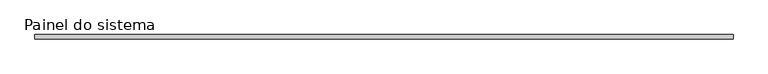
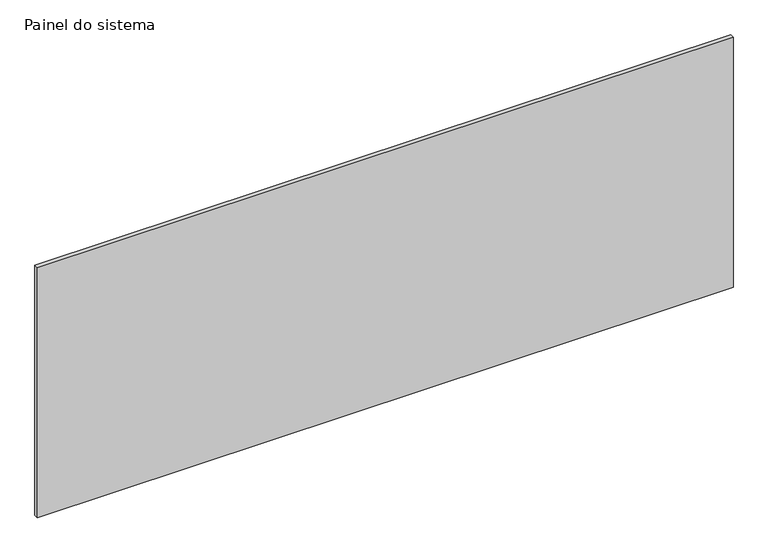
"""IFC4 building model written with IfcOpenShell, lengths in millimetres: plate geometry, Painel do sistema : Envidraçado."""

from ifc_helpers import new_model, si_unit, origin, origin_with_axes, place, context, project, spatial, polyline, outline, extrude, source, transform, mapped, element, save


def painel_do_sistema_4da26680(model_context):
    return source(origin(), model_context, "Body", "SweptSolid", [
        extrude(outline(polyline([(1975.0000075, 24.5), (-1975.0000075, 24.5), (-1975.0000075, 49.5), (1975.0000075, 49.5), (1975.0000075, 24.5)])), origin_with_axes(), (0.0, 0.0, 1.0), 1500.0),
    ])


if __name__ == "__main__":
    model = new_model("IFC4")
    model_context = context("Model", 3, world=origin())
    ifc_project = project(units=[si_unit("LENGTHUNIT", "METRE", prefix="MILLI")], contexts=[model_context])
    site = spatial("IfcSite", under=ifc_project)
    building = spatial("IfcBuilding", under=site)
    placement = place(None, origin())
    painel_do_sistema_shape = painel_do_sistema_4da26680(model_context)
    element("IfcPlate", 1, ObjectType="Painel do sistema : Envidraçado", at=placement, inside=building, context=model_context, shape_type="MappedRepresentation", body=[
        mapped(painel_do_sistema_shape, transform((0.0, 0.0, 0.0), x_axis=(1.0, 0.0, 0.0), y_axis=(0.0, 1.0, 0.0), z_axis=(0.0, 0.0, 1.0))),
    ])
    save(model, "model.ifc")

# Revit data of these elements
# Type "Painel do sistema : Envidraçado"
#   Construction Type Id = "GSP4R"
#   Analytic Construction = "Vidraça única Pilkington 1/8 pol"
#   Visual Light Transmittance = 0.9
#   Solar Heat Gain Coefficient = 0.86
#   Heat Transfer Coefficient (U) = 6.7069 W/(m²·K)
# Element 1 (IfcPlate, "Painel do sistema : Envidraçado")
#   Materials on its faces: "Vidro"
# Materials
#   "Vidro": class "Vidro", colour RGB 0 128 192, transparency 0.9, Description = "Vidro de sílica", Cost = 0
